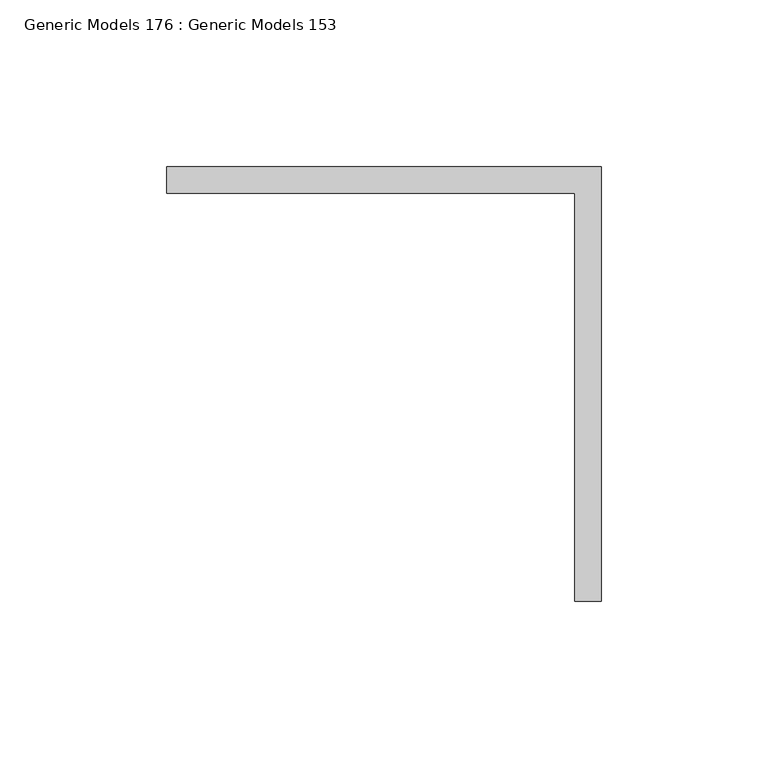
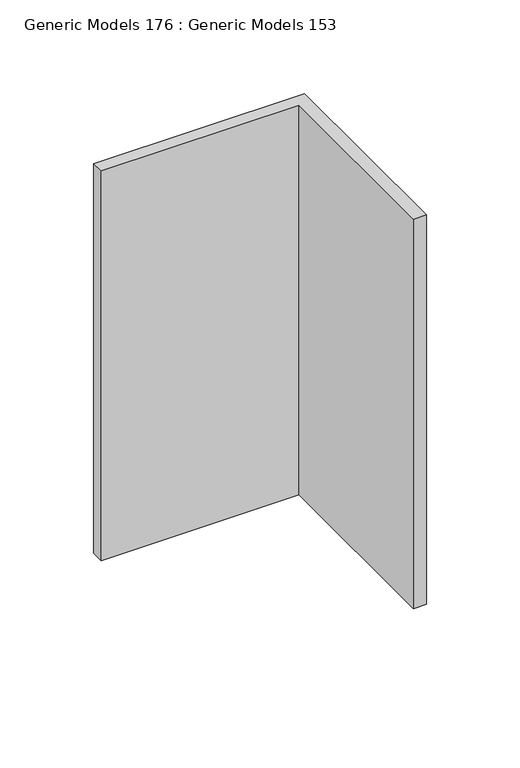
"""IFC4 building model written with IfcOpenShell, lengths in millimetres: proxy geometry, Generic Models 176 : Generic Models 153."""

from ifc_helpers import new_model, si_unit, frame, origin, place, context, project, spatial, polyline, outline, extrude, source, transform, mapped, element, save


def generic_models_176_generic_models_153_e7f4059d(model_context):
    return source(origin(), model_context, "Body", "SweptSolid", [
        extrude(outline(polyline([(31762.6846032, 30574.3156612), (31762.6846032, 30696.5531612), (31640.4471032, 30696.5531612), (31640.4471032, 30704.4906612), (31770.6221032, 30704.4906612), (31770.6221032, 30574.3156612), (31762.6846032, 30574.3156612)])), frame((0.0, 0.0, 271626.0125), z_axis=(0.0, 0.0, 1.0), x_axis=(1.0, 0.0, 0.0)), (0.0, 0.0, 1.0), 254.0),
    ])


if __name__ == "__main__":
    model = new_model("IFC4")
    model_context = context("Model", 3, world=origin())
    ifc_project = project(units=[si_unit("LENGTHUNIT", "METRE", prefix="MILLI")], contexts=[model_context])
    site = spatial("IfcSite", under=ifc_project)
    building = spatial("IfcBuilding", under=site)
    placement = place(None, origin())
    generic_models_176_generic_models_153_shape = generic_models_176_generic_models_153_e7f4059d(model_context)
    element("IfcBuildingElementProxy", 1, Name="Generic Models 176 : Generic Models 153", ObjectType="Generic Models 176 : Generic Models 153", at=placement, inside=building, context=model_context, shape_type="MappedRepresentation", body=[
        mapped(generic_models_176_generic_models_153_shape, transform((0.0, 0.0, 0.0), x_axis=(1.0, 0.0, 0.0), y_axis=(0.0, 1.0, 0.0), z_axis=(0.0, 0.0, 1.0))),
    ])
    save(model, "model.ifc")
